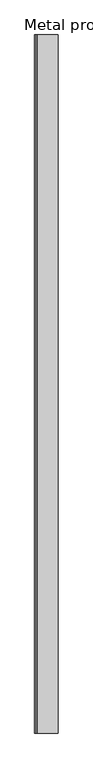
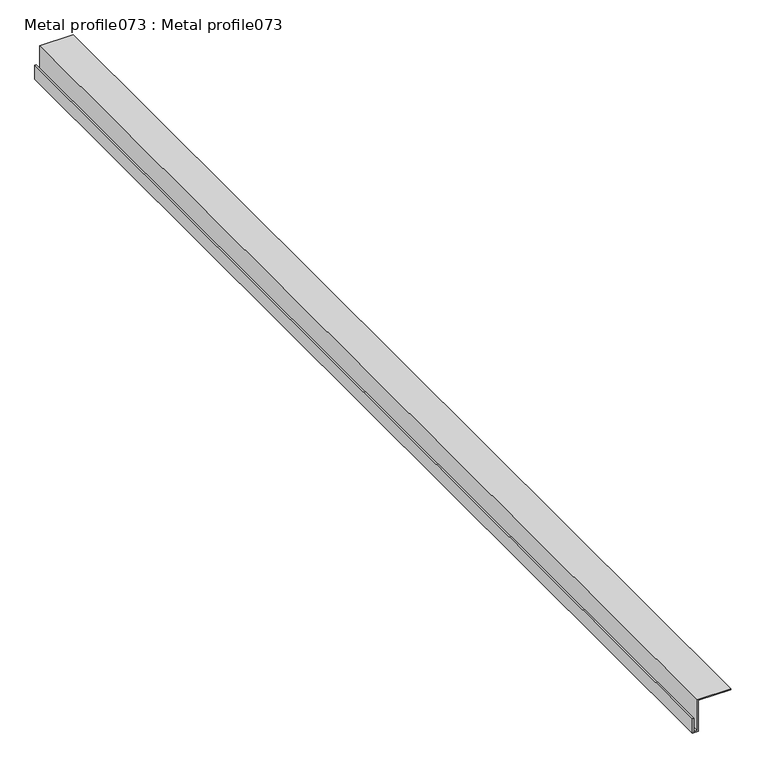
"""IFC4 building model written with IfcOpenShell, lengths in millimetres: proxy geometry, Metal profile073 : Metal profile073."""

from ifc_helpers import new_model, si_unit, frame, origin, place, context, project, spatial, polyline, outline, extrude, source, transform, mapped, element, save


def metal_profile073_metal_profile073_a0e008a6(model_context):
    return source(origin(), model_context, "Body", "SweptSolid", [
        extrude(outline(polyline([(43462.0546875, -6438.5234375), (43462.0546875, -6428.0600586), (43519.1640625, -6428.0600586), (43519.1640625, -6371.3837891), (43521.1640625, -6371.3837891), (43521.1640625, -6430.0600586), (43464.0546875, -6430.0600586), (43464.0546875, -6436.5234375), (43488.4296875, -6436.5234375), (43488.4296875, -6438.5234375), (43462.0546875, -6438.5234375)])), frame((0.0, 7982.1531721, 0.0), z_axis=(0.0, 1.0, 0.0), x_axis=(0.0, 0.0, 1.0)), (0.0, 0.0, 1.0), 2000.0),
    ])


if __name__ == "__main__":
    model = new_model("IFC4")
    model_context = context("Model", 3, world=origin())
    ifc_project = project(units=[si_unit("LENGTHUNIT", "METRE", prefix="MILLI")], contexts=[model_context])
    site = spatial("IfcSite", under=ifc_project)
    building = spatial("IfcBuilding", under=site)
    placement = place(None, origin())
    metal_profile073_metal_profile073_shape = metal_profile073_metal_profile073_a0e008a6(model_context)
    element("IfcBuildingElementProxy", 1, Name="Metal profile073 : Metal profile073", ObjectType="Metal profile073 : Metal profile073", at=placement, inside=building, context=model_context, shape_type="MappedRepresentation", body=[
        mapped(metal_profile073_metal_profile073_shape, transform((0.0, 0.0, 0.0), x_axis=(1.0, 0.0, 0.0), y_axis=(0.0, 1.0, 0.0), z_axis=(0.0, 0.0, 1.0))),
    ])
    save(model, "model.ifc")

# Revit data of these elements
# Type "Metal profile073 : Metal profile073"
#   NameOverride = "Metal profile073"
# Element 1 (IfcBuildingElementProxy, "Metal profile073 : Metal profile073")
#   Materials on its faces: "ANGLE TRIM"
# Materials
#   "ANGLE TRIM": class "Unassigned", colour RGB 250 255 0, transparency 0
